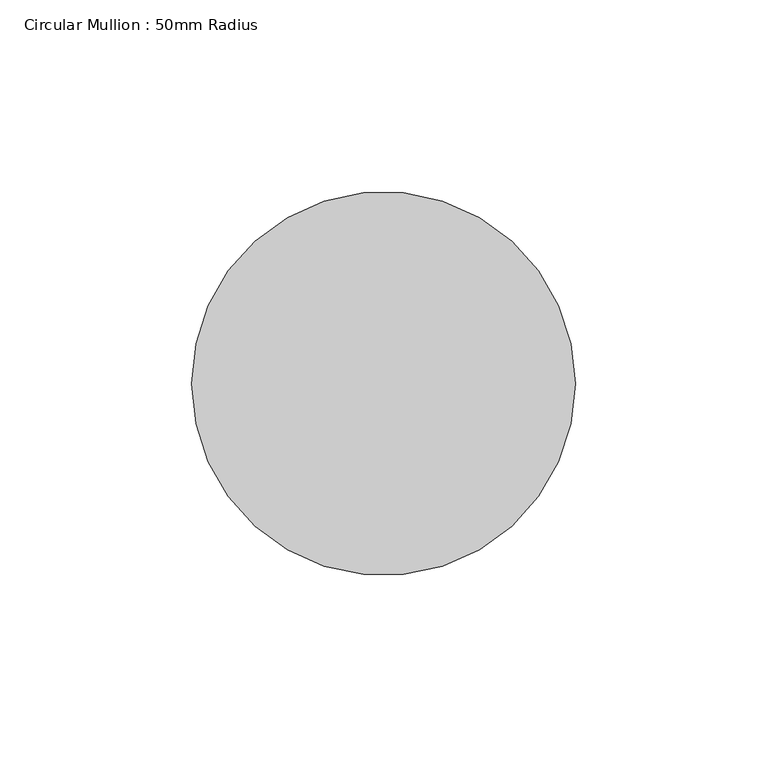
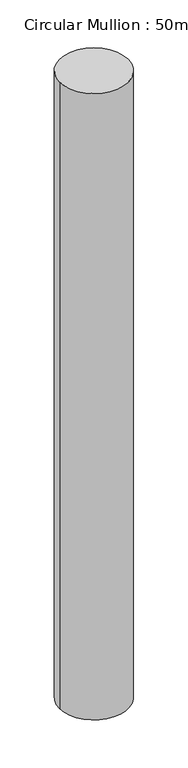
"""IFC4 building model written with IfcOpenShell, lengths in millimetres: member geometry, Circular Mullion : 50mm Radius."""

import ifcopenshell
import ifcopenshell.guid

model = None  # the IFC model being written
_history = None  # IfcOwnerHistory: only IFC2X3 demands one
_inside = {}  # id of a spatial element -> (the spatial element, [elements in it])
_under = {}  # id of a project, library or spatial element -> (it, [spatial elements below it])
_declared = {}  # id of a project -> (the project, [libraries it declares])
_typed = {}  # id of a type object -> (the type object, [elements of that type])
_made_of = {}  # id of a material, layer set ... -> (it, [elements and type objects made of it])


def new_model(schema):
    """Start an empty IFC model of exactly this schema.

    Asked for "IFC4X3", IfcOpenShell would pick the latest addendum, in which some entities
    have other attributes; the version numbers below select the first issue.
    IFC2X3 requires an IfcOwnerHistory on every rooted entity: one is made here for all.
    """
    global model, _history
    if schema == "IFC4X3":
        model = ifcopenshell.file(schema_version=(4, 3, 0, 0))
    else:
        model = ifcopenshell.file(schema=schema)
    _inside.clear()
    _under.clear()
    _declared.clear()
    _typed.clear()
    _made_of.clear()
    _history = None
    if model.schema == "IFC2X3":
        org = make("IfcOrganization", Name="unknown")
        user = make(
            "IfcPersonAndOrganization",
            ThePerson=make("IfcPerson", FamilyName="unknown"),
            TheOrganization=org,
        )
        app = make(
            "IfcApplication",
            ApplicationDeveloper=org,
            Version="unknown",
            ApplicationFullName="unknown",
            ApplicationIdentifier="unknown",
        )
        _history = make(
            "IfcOwnerHistory",
            OwningUser=user,
            OwningApplication=app,
            ChangeAction="ADDED",
            CreationDate=0,
        )
    return model


def make(cls, **values):
    """One entity of the class cls with the attributes given. An attribute that is None is left unset."""
    return model.create_entity(
        cls, **{name: value for name, value in values.items() if value is not None}
    )


def rooted(cls, **values):
    """An entity with a GlobalId (a new one), such as an element, a storey or a relation."""
    return make(cls, GlobalId=ifcopenshell.guid.new(), OwnerHistory=_history, **values)


def si_unit(unit_type, name, prefix=None):
    """IfcSIUnit, for example si_unit("LENGTHUNIT", "METRE", prefix="MILLI")."""
    return make("IfcSIUnit", UnitType=unit_type, Prefix=prefix, Name=name)


def assignment(units):
    """IfcUnitAssignment: the units of a project."""
    return None if units is None else make("IfcUnitAssignment", Units=units)


def point(xyz):
    """IfcCartesianPoint."""
    return None if xyz is None else make("IfcCartesianPoint", Coordinates=xyz)


def direction(xyz):
    """IfcDirection."""
    return None if xyz is None else make("IfcDirection", DirectionRatios=xyz)


def frame(location, z_axis=None, x_axis=None):
    """IfcAxis2Placement3D, a coordinate frame: its origin and axes. An axis left out is left unset."""
    return make(
        "IfcAxis2Placement3D",
        Location=point(location),
        Axis=direction(z_axis),
        RefDirection=direction(x_axis),
    )


def frame_2d(location, x_axis=None):
    """IfcAxis2Placement2D, a coordinate frame in the plane: its origin and x axis."""
    return make(
        "IfcAxis2Placement2D", Location=point(location), RefDirection=direction(x_axis)
    )


def origin():
    """The frame at (0, 0, 0) with its axes left unset."""
    return frame((0.0, 0.0, 0.0))


def origin_2d():
    """The frame at (0, 0) in the plane with its x axis left unset."""
    return frame_2d((0.0, 0.0))


def place(relative_to, where):
    """IfcLocalPlacement: puts the frame where relative to a parent placement (None: the world)."""
    return make(
        "IfcLocalPlacement", PlacementRelTo=relative_to, RelativePlacement=where
    )


def context(
    kind, dimensions, precision=None, world=None, true_north=None, identifier=None
):
    """IfcGeometricRepresentationContext, for example the 3D "Model" context."""
    return make(
        "IfcGeometricRepresentationContext",
        ContextIdentifier=identifier,
        ContextType=kind,
        CoordinateSpaceDimension=dimensions,
        Precision=precision,
        WorldCoordinateSystem=world,
        TrueNorth=true_north,
    )


def project(units=None, contexts=None):
    """IfcProject with its units and contexts."""
    return rooted(
        "IfcProject",
        Name="project",
        RepresentationContexts=contexts,
        UnitsInContext=assignment(units),
    )


def spatial(cls, under=None, at=None, **own):
    """A site, building, storey or space (cls), placed at a placement, below another one or the project."""
    s = rooted(cls, ObjectPlacement=at, **own)
    if under is not None:
        _under.setdefault(under.id(), (under, []))[1].append(s)
    return s


def circle_curve(where, radius):
    """IfcCircle in the frame where."""
    return make("IfcCircle", Position=where, Radius=radius)


def trimmed(basis, trim1, trim2, sense, master):
    """IfcTrimmedCurve: the piece of a basis curve between two trims."""
    return make(
        "IfcTrimmedCurve",
        BasisCurve=basis,
        Trim1=trim1,
        Trim2=trim2,
        SenseAgreement=sense,
        MasterRepresentation=master,
    )


def segment(curve, same_sense, transition):
    """IfcCompositeCurveSegment."""
    return make(
        "IfcCompositeCurveSegment",
        Transition=transition,
        SameSense=same_sense,
        ParentCurve=curve,
    )


def composite_curve(segments, self_intersect=None):
    """IfcCompositeCurve: segments joined end to end."""
    return make("IfcCompositeCurve", Segments=segments, SelfIntersect=self_intersect)


def outline(outer, holes=None, kind="AREA"):
    """IfcArbitraryClosedProfileDef: a profile drawn as a closed curve; with holes, ...WithVoids."""
    if holes is None:
        return make("IfcArbitraryClosedProfileDef", ProfileType=kind, OuterCurve=outer)
    return make(
        "IfcArbitraryProfileDefWithVoids",
        ProfileType=kind,
        OuterCurve=outer,
        InnerCurves=holes,
    )


def extrude(swept, where, along, depth):
    """IfcExtrudedAreaSolid: the profile swept, set in the frame where, extruded along a direction by depth."""
    return make(
        "IfcExtrudedAreaSolid",
        SweptArea=swept,
        Position=where,
        ExtrudedDirection=direction(along),
        Depth=depth,
    )


def shape(context_of_items, identifier, shape_type, items):
    """IfcShapeRepresentation: the items that make up one representation, for example the "Body"."""
    return make(
        "IfcShapeRepresentation",
        ContextOfItems=context_of_items,
        RepresentationIdentifier=identifier,
        RepresentationType=shape_type,
        Items=items,
    )


def source(mapping_origin, context_of_items, identifier, shape_type, items):
    """IfcRepresentationMap: a shape defined once, which mapped items show again and again."""
    return make(
        "IfcRepresentationMap",
        MappingOrigin=mapping_origin,
        MappedRepresentation=shape(context_of_items, identifier, shape_type, items),
    )


def transform(
    local_origin,
    x_axis=None,
    y_axis=None,
    z_axis=None,
    scale=None,
    scale2=None,
    scale3=None,
    uniform=True,
):
    """IfcCartesianTransformationOperator3D, or its non-uniform kind. x_axis, y_axis, z_axis: its Axis1, 2, 3."""
    if uniform:
        return make(
            "IfcCartesianTransformationOperator3D",
            Axis1=direction(x_axis),
            Axis2=direction(y_axis),
            LocalOrigin=point(local_origin),
            Scale=scale,
            Axis3=direction(z_axis),
        )
    return make(
        "IfcCartesianTransformationOperator3DnonUniform",
        Axis1=direction(x_axis),
        Axis2=direction(y_axis),
        LocalOrigin=point(local_origin),
        Scale=scale,
        Axis3=direction(z_axis),
        Scale2=scale2,
        Scale3=scale3,
    )


def mapped(mapping_source, mapping_target):
    """IfcMappedItem: shows the shape of a source again, moved by a transform."""
    return make(
        "IfcMappedItem", MappingSource=mapping_source, MappingTarget=mapping_target
    )


def made_of(thing, what):
    """Note that an element or type object is made of a material, layer set ...; save() writes the relation."""
    if what is not None:
        _made_of.setdefault(what.id(), (what, []))[1].append(thing)
    return thing


def element(
    cls,
    number,
    at=None,
    inside=None,
    cuts=None,
    type_object=None,
    material=None,
    context=None,
    identifier="Body",
    shape_type=None,
    held_by="IfcProductDefinitionShape",
    body=None,
    shapes=None,
    **own,
):
    """One element of the class cls, such as IfcWall. Its Tag is "e" and its number.

    at: its placement. inside: the storey or other place that contains it. cuts: it is an
    opening in that element (IfcRelVoidsElement). A single representation is given by context,
    identifier, shape_type and body (its items); several are given by shapes. held_by: the class
    of the entity that holds the representations. save() writes the other relations.
    """
    e = rooted(cls, Tag="e%d" % number, ObjectPlacement=at, **own)
    if body is not None:
        shapes = [shape(context, identifier, shape_type, body)]
    if shapes is not None:
        e.Representation = make(held_by, Representations=shapes)
    if inside is not None:
        _inside.setdefault(inside.id(), (inside, []))[1].append(e)
    if cuts is not None:
        rooted(
            "IfcRelVoidsElement", RelatingBuildingElement=cuts, RelatedOpeningElement=e
        )
    if type_object is not None:
        _typed.setdefault(type_object.id(), (type_object, []))[1].append(e)
    return made_of(e, material)


def aggregate(whole, parts):
    """IfcRelAggregates: a whole, such as a stair, and the parts it consists of."""
    return rooted("IfcRelAggregates", RelatingObject=whole, RelatedObjects=parts)


def save(model, path):
    """Write the relations noted so far, then the file.

    IfcRelAggregates (storeys below a building ...), IfcRelContainedInSpatialStructure (elements
    in a storey), IfcRelDefinesByType, IfcRelAssociatesMaterial and IfcRelDeclares: one each for
    every whole, place, type object, material and project.
    """
    for whole, parts in _under.values():
        aggregate(whole, parts)
    for where, things in _inside.values():
        rooted(
            "IfcRelContainedInSpatialStructure",
            RelatedElements=things,
            RelatingStructure=where,
        )
    for kind, things in _typed.values():
        rooted("IfcRelDefinesByType", RelatedObjects=things, RelatingType=kind)
    for what, things in _made_of.values():
        rooted("IfcRelAssociatesMaterial", RelatedObjects=things, RelatingMaterial=what)
    for by, libraries in _declared.values():
        rooted("IfcRelDeclares", RelatingContext=by, RelatedDefinitions=libraries)
    model.write(path)


def circular_mullion_50mm_radius_c8180037(model_context):
    return source(origin(), model_context, "Body", "SweptSolid", [
        extrude(outline(composite_curve([segment(trimmed(circle_curve(origin_2d(), 50.0), [point((50.0, 0.0))], [point((-50.0, 0.0))], False, "CARTESIAN"), True, "CONTINUOUS"), segment(trimmed(circle_curve(origin_2d(), 50.0), [point((-50.0, 0.0))], [point((50.0, 0.0))], False, "CARTESIAN"), True, "CONTINUOUS")], self_intersect=False)), frame((0.0, 0.0, -964.051897), z_axis=(0.0, 0.0, 1.0), x_axis=(1.0, 0.0, 0.0)), (0.0, 0.0, 1.0), 964.051897),
    ])


if __name__ == "__main__":
    model = new_model("IFC4")
    model_context = context("Model", 3, world=origin())
    ifc_project = project(units=[si_unit("LENGTHUNIT", "METRE", prefix="MILLI")], contexts=[model_context])
    site = spatial("IfcSite", under=ifc_project)
    building = spatial("IfcBuilding", under=site)
    placement = place(None, origin())
    circular_mullion_50mm_radius_shape = circular_mullion_50mm_radius_c8180037(model_context)
    element("IfcMember", 1, ObjectType="Circular Mullion : 50mm Radius", at=placement, inside=building, context=model_context, shape_type="MappedRepresentation", body=[
        mapped(circular_mullion_50mm_radius_shape, transform((0.0, 0.0, 0.0), x_axis=(1.0, 0.0, 0.0), y_axis=(0.0, 1.0, 0.0), z_axis=(0.0, 0.0, 1.0))),
    ])
    save(model, "model.ifc")

# Revit data of these elements
# Type "Circular Mullion : 50mm Radius"
#   built-in parameter 1007350 = 0.164042 (stored number, unit not read)
# Element 1 (IfcMember, "Circular Mullion : 50mm Radius")
#   Materials on its faces: "Aluminium"
# Materials
#   "Aluminium": class "Metal", colour RGB 247 247 247, transparency 0, Description = "Aluminium 6061", Cost = 0
